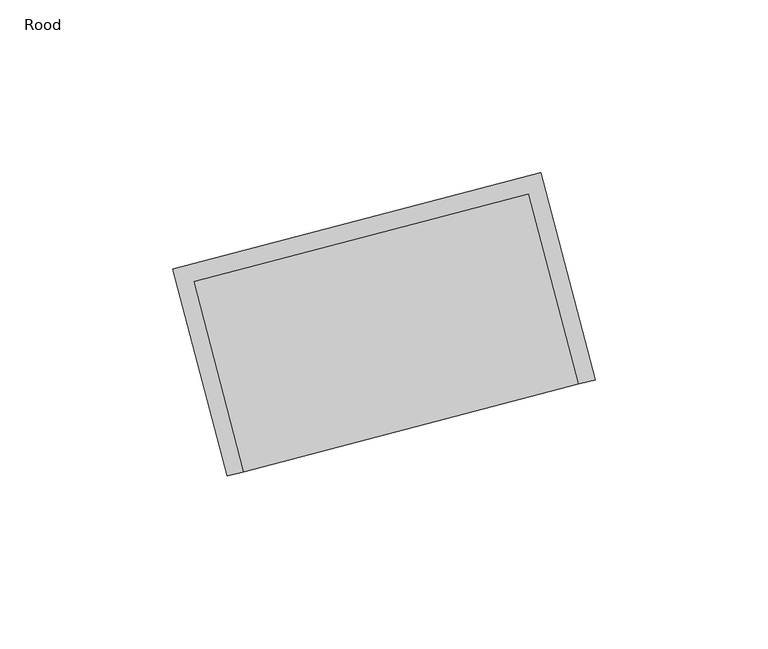
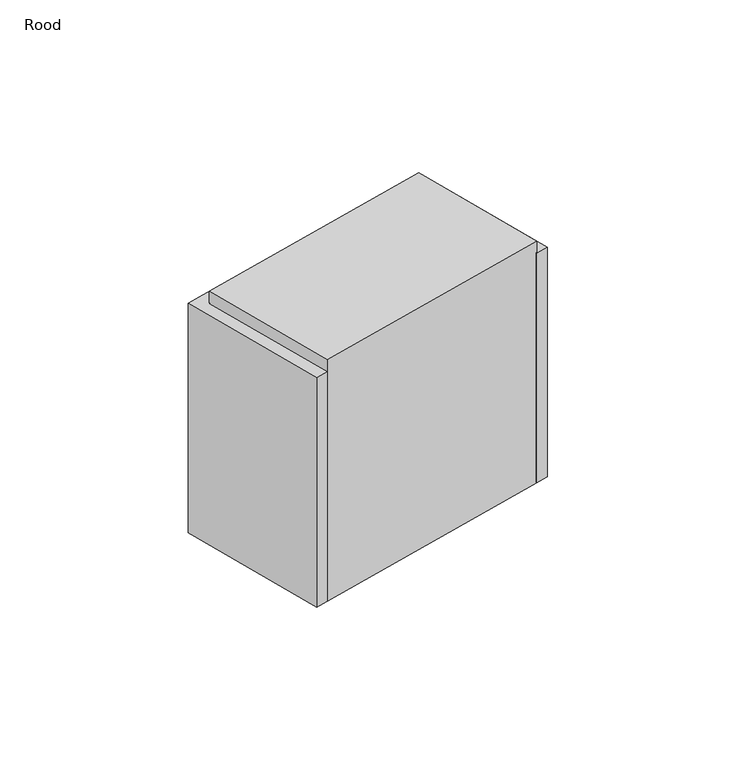
"""IFC4 building model written with IfcOpenShell, lengths in millimetres: proxy geometry, 00_GMA_steen_versie_6 : Rood."""

from ifc_helpers import new_model, si_unit, origin, origin_with_axes, place, context, project, spatial, polyline, outline, extrude, source, transform, mapped, element, save


def rood_2ddd8018(model_context):
    return source(origin(), model_context, "Body", "SweptSolid", [
        extrude(outline(polyline([(24.8461542, 24.0369432), (9.1731432, 83.919349), (115.5141152, 111.7519519), (131.1871262, 51.8695461), (126.3500577, 50.6035411), (111.9430518, 105.6488784), (15.2762167, 80.3482856), (29.6832226, 25.3029482), (24.8461542, 24.0369432)])), origin_with_axes(), (0.0, 0.0, 1.0), 95.0),
        extrude(outline(polyline([(111.9430518, 105.6488784), (126.3500577, 50.6035411), (29.6832226, 25.3029482), (15.2762167, 80.3482856), (111.9430518, 105.6488784)])), origin_with_axes(), (0.0, 0.0, 1.0), 100.0),
    ])


if __name__ == "__main__":
    model = new_model("IFC4")
    model_context = context("Model", 3, world=origin())
    ifc_project = project(units=[si_unit("LENGTHUNIT", "METRE", prefix="MILLI")], contexts=[model_context])
    site = spatial("IfcSite", under=ifc_project)
    building = spatial("IfcBuilding", under=site)
    placement = place(None, origin())
    rood_shape = rood_2ddd8018(model_context)
    element("IfcBuildingElementProxy", 1, Name="00_GMA_steen_versie_6 : Rood", ObjectType="00_GMA_steen_versie_6 : Rood", at=placement, inside=building, context=model_context, shape_type="MappedRepresentation", body=[
        mapped(rood_shape, transform((0.0, 0.0, 0.0), x_axis=(1.0, 0.0, 0.0), y_axis=(0.0, 1.0, 0.0), z_axis=(0.0, 0.0, 1.0))),
    ])
    save(model, "model.ifc")

# Revit data of these elements
# Type "00_GMA_steen_versie_6 : Rood"
#   Voegdikte = 95 mm
#   VoegTovSteen = -5 mm
#   StootvoegLinksHalfOnder [instance default] = 5 mm
#   StootvoegLinksHalfBoven [instance default] = 5 mm
#   StootVoegRechtsHalfOnder [instance default] = 5 mm
#   StootVoegRechtsHalfBoven [instance default] = 5 mm
#   StootVoegBreedteRechts [instance default] = 10 mm
#   StootVoegBreedteLinks [instance default] = 10 mm
#   Steendikte = 100 mm
#   LintVoegOnderHalf [instance default] = 0 mm
#   LintVoegOnder [instance default] = 0 mm
#   LintVoegBovenHalf [instance default] = 5 mm
#   LintVoegBoven [instance default] = 10 mm
#   materiaal = 21_steen_rood
#   MateriaalVoeg = 20_voeg
#   Default Elevation = 0
# Element 1 (IfcBuildingElementProxy, "00_GMA_steen_versie_6 : Rood")
#   Materials on its faces: "20_voeg", "21_steen_rood"
# Materials
#   "21_steen_rood": class "Unassigned", colour RGB 213 111 43, transparency 0, Cost = 0
#   "20_voeg": class "Concrete", colour RGB 86 86 86, transparency 0, Manufacturer = "RevitGG", URL = "www.revitgg.nl", Description = "zandcement, generiek materiaal", Cost = 0
